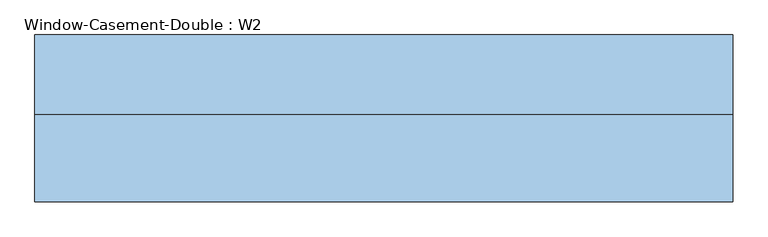
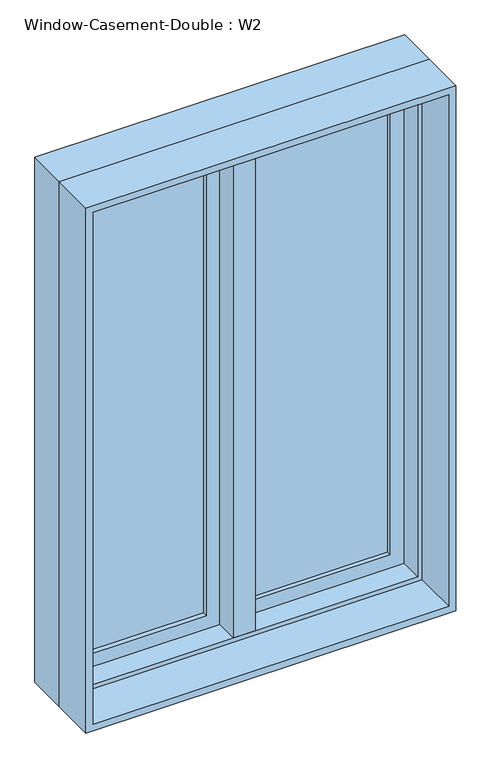
"""IFC4 building model written with IfcOpenShell, lengths in millimetres: window geometry, Window-Casement-Double : W2."""

import ifcopenshell
import ifcopenshell.guid

model = None  # the IFC model being written
_history = None  # IfcOwnerHistory: only IFC2X3 demands one
_inside = {}  # id of a spatial element -> (the spatial element, [elements in it])
_under = {}  # id of a project, library or spatial element -> (it, [spatial elements below it])
_declared = {}  # id of a project -> (the project, [libraries it declares])
_typed = {}  # id of a type object -> (the type object, [elements of that type])
_made_of = {}  # id of a material, layer set ... -> (it, [elements and type objects made of it])


def new_model(schema):
    """Start an empty IFC model of exactly this schema.

    Asked for "IFC4X3", IfcOpenShell would pick the latest addendum, in which some entities
    have other attributes; the version numbers below select the first issue.
    IFC2X3 requires an IfcOwnerHistory on every rooted entity: one is made here for all.
    """
    global model, _history
    if schema == "IFC4X3":
        model = ifcopenshell.file(schema_version=(4, 3, 0, 0))
    else:
        model = ifcopenshell.file(schema=schema)
    _inside.clear()
    _under.clear()
    _declared.clear()
    _typed.clear()
    _made_of.clear()
    _history = None
    if model.schema == "IFC2X3":
        org = make("IfcOrganization", Name="unknown")
        user = make(
            "IfcPersonAndOrganization",
            ThePerson=make("IfcPerson", FamilyName="unknown"),
            TheOrganization=org,
        )
        app = make(
            "IfcApplication",
            ApplicationDeveloper=org,
            Version="unknown",
            ApplicationFullName="unknown",
            ApplicationIdentifier="unknown",
        )
        _history = make(
            "IfcOwnerHistory",
            OwningUser=user,
            OwningApplication=app,
            ChangeAction="ADDED",
            CreationDate=0,
        )
    return model


def make(cls, **values):
    """One entity of the class cls with the attributes given. An attribute that is None is left unset."""
    return model.create_entity(
        cls, **{name: value for name, value in values.items() if value is not None}
    )


def rooted(cls, **values):
    """An entity with a GlobalId (a new one), such as an element, a storey or a relation."""
    return make(cls, GlobalId=ifcopenshell.guid.new(), OwnerHistory=_history, **values)


def si_unit(unit_type, name, prefix=None):
    """IfcSIUnit, for example si_unit("LENGTHUNIT", "METRE", prefix="MILLI")."""
    return make("IfcSIUnit", UnitType=unit_type, Prefix=prefix, Name=name)


def assignment(units):
    """IfcUnitAssignment: the units of a project."""
    return None if units is None else make("IfcUnitAssignment", Units=units)


def point(xyz):
    """IfcCartesianPoint."""
    return None if xyz is None else make("IfcCartesianPoint", Coordinates=xyz)


def direction(xyz):
    """IfcDirection."""
    return None if xyz is None else make("IfcDirection", DirectionRatios=xyz)


def frame(location, z_axis=None, x_axis=None):
    """IfcAxis2Placement3D, a coordinate frame: its origin and axes. An axis left out is left unset."""
    return make(
        "IfcAxis2Placement3D",
        Location=point(location),
        Axis=direction(z_axis),
        RefDirection=direction(x_axis),
    )


def origin():
    """The frame at (0, 0, 0) with its axes left unset."""
    return frame((0.0, 0.0, 0.0))


def place(relative_to, where):
    """IfcLocalPlacement: puts the frame where relative to a parent placement (None: the world)."""
    return make(
        "IfcLocalPlacement", PlacementRelTo=relative_to, RelativePlacement=where
    )


def context(
    kind, dimensions, precision=None, world=None, true_north=None, identifier=None
):
    """IfcGeometricRepresentationContext, for example the 3D "Model" context."""
    return make(
        "IfcGeometricRepresentationContext",
        ContextIdentifier=identifier,
        ContextType=kind,
        CoordinateSpaceDimension=dimensions,
        Precision=precision,
        WorldCoordinateSystem=world,
        TrueNorth=true_north,
    )


def project(units=None, contexts=None):
    """IfcProject with its units and contexts."""
    return rooted(
        "IfcProject",
        Name="project",
        RepresentationContexts=contexts,
        UnitsInContext=assignment(units),
    )


def spatial(cls, under=None, at=None, **own):
    """A site, building, storey or space (cls), placed at a placement, below another one or the project."""
    s = rooted(cls, ObjectPlacement=at, **own)
    if under is not None:
        _under.setdefault(under.id(), (under, []))[1].append(s)
    return s


def polyline(points):
    """IfcPolyline through the points."""
    return make("IfcPolyline", Points=[point(p) for p in points])


def outline(outer, holes=None, kind="AREA"):
    """IfcArbitraryClosedProfileDef: a profile drawn as a closed curve; with holes, ...WithVoids."""
    if holes is None:
        return make("IfcArbitraryClosedProfileDef", ProfileType=kind, OuterCurve=outer)
    return make(
        "IfcArbitraryProfileDefWithVoids",
        ProfileType=kind,
        OuterCurve=outer,
        InnerCurves=holes,
    )


def extrude(swept, where, along, depth):
    """IfcExtrudedAreaSolid: the profile swept, set in the frame where, extruded along a direction by depth."""
    return make(
        "IfcExtrudedAreaSolid",
        SweptArea=swept,
        Position=where,
        ExtrudedDirection=direction(along),
        Depth=depth,
    )


def faces_of(points, faces, orient=None, outer=None):
    """IfcFace entities. A face is a list of loops; a loop is a list of indices into points, from 0.

    orient and outer hold one flag for each loop. By default every Orientation is true, the
    first loop of a face is its IfcFaceOuterBound and the others are IfcFaceBound.
    """
    made = []
    for i, loops in enumerate(faces):
        bounds = []
        for j, loop in enumerate(loops):
            is_outer = j == 0 if outer is None else outer[i][j]
            bounds.append(
                make(
                    "IfcFaceOuterBound" if is_outer else "IfcFaceBound",
                    Bound=make("IfcPolyLoop", Polygon=[points[k] for k in loop]),
                    Orientation=True if orient is None else orient[i][j],
                )
            )
        made.append(make("IfcFace", Bounds=bounds))
    return made


def faceted_brep(points, faces, orient=None, outer=None, voids=None):
    """IfcFacetedBrep: a solid bounded by flat faces; with voids (closed shells), ...WithVoids."""
    shared = [point(p) for p in points]
    hull = make("IfcClosedShell", CfsFaces=faces_of(shared, faces, orient, outer))
    if voids is None:
        return make("IfcFacetedBrep", Outer=hull)
    return make(
        "IfcFacetedBrepWithVoids",
        Outer=hull,
        Voids=[
            make(cls, CfsFaces=faces_of(shared, fs, o, b)) for cls, fs, o, b in voids
        ],
    )


def shape(context_of_items, identifier, shape_type, items):
    """IfcShapeRepresentation: the items that make up one representation, for example the "Body"."""
    return make(
        "IfcShapeRepresentation",
        ContextOfItems=context_of_items,
        RepresentationIdentifier=identifier,
        RepresentationType=shape_type,
        Items=items,
    )


def source(mapping_origin, context_of_items, identifier, shape_type, items):
    """IfcRepresentationMap: a shape defined once, which mapped items show again and again."""
    return make(
        "IfcRepresentationMap",
        MappingOrigin=mapping_origin,
        MappedRepresentation=shape(context_of_items, identifier, shape_type, items),
    )


def transform(
    local_origin,
    x_axis=None,
    y_axis=None,
    z_axis=None,
    scale=None,
    scale2=None,
    scale3=None,
    uniform=True,
):
    """IfcCartesianTransformationOperator3D, or its non-uniform kind. x_axis, y_axis, z_axis: its Axis1, 2, 3."""
    if uniform:
        return make(
            "IfcCartesianTransformationOperator3D",
            Axis1=direction(x_axis),
            Axis2=direction(y_axis),
            LocalOrigin=point(local_origin),
            Scale=scale,
            Axis3=direction(z_axis),
        )
    return make(
        "IfcCartesianTransformationOperator3DnonUniform",
        Axis1=direction(x_axis),
        Axis2=direction(y_axis),
        LocalOrigin=point(local_origin),
        Scale=scale,
        Axis3=direction(z_axis),
        Scale2=scale2,
        Scale3=scale3,
    )


def mapped(mapping_source, mapping_target):
    """IfcMappedItem: shows the shape of a source again, moved by a transform."""
    return make(
        "IfcMappedItem", MappingSource=mapping_source, MappingTarget=mapping_target
    )


def made_of(thing, what):
    """Note that an element or type object is made of a material, layer set ...; save() writes the relation."""
    if what is not None:
        _made_of.setdefault(what.id(), (what, []))[1].append(thing)
    return thing


def element(
    cls,
    number,
    at=None,
    inside=None,
    cuts=None,
    type_object=None,
    material=None,
    context=None,
    identifier="Body",
    shape_type=None,
    held_by="IfcProductDefinitionShape",
    body=None,
    shapes=None,
    **own,
):
    """One element of the class cls, such as IfcWall. Its Tag is "e" and its number.

    at: its placement. inside: the storey or other place that contains it. cuts: it is an
    opening in that element (IfcRelVoidsElement). A single representation is given by context,
    identifier, shape_type and body (its items); several are given by shapes. held_by: the class
    of the entity that holds the representations. save() writes the other relations.
    """
    e = rooted(cls, Tag="e%d" % number, ObjectPlacement=at, **own)
    if body is not None:
        shapes = [shape(context, identifier, shape_type, body)]
    if shapes is not None:
        e.Representation = make(held_by, Representations=shapes)
    if inside is not None:
        _inside.setdefault(inside.id(), (inside, []))[1].append(e)
    if cuts is not None:
        rooted(
            "IfcRelVoidsElement", RelatingBuildingElement=cuts, RelatedOpeningElement=e
        )
    if type_object is not None:
        _typed.setdefault(type_object.id(), (type_object, []))[1].append(e)
    return made_of(e, material)


def aggregate(whole, parts):
    """IfcRelAggregates: a whole, such as a stair, and the parts it consists of."""
    return rooted("IfcRelAggregates", RelatingObject=whole, RelatedObjects=parts)


def save(model, path):
    """Write the relations noted so far, then the file.

    IfcRelAggregates (storeys below a building ...), IfcRelContainedInSpatialStructure (elements
    in a storey), IfcRelDefinesByType, IfcRelAssociatesMaterial and IfcRelDeclares: one each for
    every whole, place, type object, material and project.
    """
    for whole, parts in _under.values():
        aggregate(whole, parts)
    for where, things in _inside.values():
        rooted(
            "IfcRelContainedInSpatialStructure",
            RelatedElements=things,
            RelatingStructure=where,
        )
    for kind, things in _typed.values():
        rooted("IfcRelDefinesByType", RelatedObjects=things, RelatingType=kind)
    for what, things in _made_of.values():
        rooted("IfcRelAssociatesMaterial", RelatedObjects=things, RelatingMaterial=what)
    for by, libraries in _declared.values():
        rooted("IfcRelDeclares", RelatingContext=by, RelatedDefinitions=libraries)
    model.write(path)


def window_casement_double_w2_23809e8b(model_context):
    return source(origin(), model_context, "Body", "SolidModel", [
        faceted_brep([(9.525, 129.05, 2401.7), (-9.525, 129.05, 2401.7), (-9.525, 78.25, 2401.7), (9.525, 78.25, 2401.7), (9.525, 129.05, 927.1), (9.525, 78.25, 927.1), (-9.525, 78.25, 927.1), (-9.525, 129.05, 927.1), (-9.525, 78.25, 946.15), (-9.525, 78.25, 2382.65), (-30.1625, 78.25, 946.15), (-30.1625, 78.25, 2382.65), (-30.1625, 14.75, 946.15), (-30.1625, 14.75, 2382.65), (30.1625, 14.75, 946.15), (30.1625, 14.75, 2382.65), (30.1625, 78.25, 946.15), (30.1625, 78.25, 2382.65), (9.525, 78.25, 946.15), (9.525, 78.25, 2382.65)], [[[0, 1, 2, 3]], [[4, 5, 6, 7]], [[1, 0, 4, 7]], [[2, 1, 7, 6, 8, 9]], [[9, 8, 10, 11]], [[11, 10, 12, 13]], [[13, 12, 14, 15]], [[15, 14, 16, 17]], [[17, 16, 18, 19]], [[0, 3, 19, 18, 5, 4]], [[18, 8, 6, 5]], [[9, 19, 3, 2]], [[8, 18, 16, 14, 12, 10]], [[19, 9, 11, 13, 15, 17]]]),
        extrude(outline(polyline([(-66.675, 110.0), (-66.675, 103.65), (-430.15, 103.65), (-430.15, 110.0), (-66.675, 110.0)])), frame((0.0, 0.0, 984.25), z_axis=(0.0, 0.0, 1.0), x_axis=(1.0, 0.0, 0.0)), (0.0, 0.0, 1.0), 1360.3),
        extrude(outline(polyline([(-430.15, 90.95), (-430.15, 97.3), (-66.675, 97.3), (-66.675, 90.95), (-430.15, 90.95)])), frame((0.0, 0.0, 984.25), z_axis=(0.0, 0.0, 1.0), x_axis=(1.0, 0.0, 0.0)), (0.0, 0.0, 1.0), 1360.3),
        extrude(outline(polyline([(430.15, 110.0), (430.15, 103.65), (66.675, 103.65), (66.675, 110.0), (430.15, 110.0)])), frame((0.0, 0.0, 984.25), z_axis=(0.0, 0.0, 1.0), x_axis=(1.0, 0.0, 0.0)), (0.0, 0.0, 1.0), 1360.3),
        extrude(outline(polyline([(66.675, 90.95), (66.675, 97.3), (430.15, 97.3), (430.15, 90.95), (66.675, 90.95)])), frame((0.0, 0.0, 984.25), z_axis=(0.0, 0.0, 1.0), x_axis=(1.0, 0.0, 0.0)), (0.0, 0.0, 1.0), 1360.3),
        extrude(outline(polyline([(2401.7, -487.3), (927.1, -487.3), (927.1, -9.525), (2401.7, -9.525), (2401.7, -487.3)]), holes=[polyline([(2344.55, -66.675), (984.25, -66.675), (984.25, -430.15), (2344.55, -430.15), (2344.55, -66.675)])]), frame((0.0, 78.25, 0.0), z_axis=(0.0, 1.0, 0.0), x_axis=(0.0, 0.0, 1.0)), (0.0, 0.0, 1.0), 44.45),
        extrude(outline(polyline([(927.1, 487.3), (2401.7, 487.3), (2401.7, 9.525), (927.1, 9.525), (927.1, 487.3)]), holes=[polyline([(984.25, 66.675), (2344.55, 66.675), (2344.55, 430.15), (984.25, 430.15), (984.25, 66.675)])]), frame((0.0, 78.25, 0.0), z_axis=(0.0, 1.0, 0.0), x_axis=(0.0, 0.0, 1.0)), (0.0, 0.0, 1.0), 44.45),
        extrude(outline(polyline([(2414.4, -500.0), (914.4, -500.0), (914.4, 500.0), (2414.4, 500.0), (2414.4, -500.0)]), holes=[polyline([(2395.35, 480.95), (933.45, 480.95), (933.45, -480.95), (2395.35, -480.95), (2395.35, 480.95)])]), frame((0.0, -110.0, 0.0), z_axis=(0.0, 1.0, 0.0), x_axis=(0.0, 0.0, 1.0)), (0.0, 0.0, 1.0), 124.75),
        faceted_brep([(468.25, 78.25, 2382.65), (468.25, 14.75, 2382.65), (-468.25, 14.75, 2382.65), (-468.25, 78.25, 2382.65), (487.3, 129.05, 2401.7), (487.3, 78.25, 2401.7), (-487.3, 78.25, 2401.7), (-487.3, 129.05, 2401.7), (500.0, 14.75, 2414.4), (500.0, 129.05, 2414.4), (-500.0, 129.05, 2414.4), (-500.0, 14.75, 2414.4), (-468.25, 14.75, 946.15), (-468.25, 78.25, 946.15), (-487.3, 78.25, 927.1), (-487.3, 129.05, 927.1), (-500.0, 129.05, 914.4), (-500.0, 14.75, 914.4), (468.25, 14.75, 946.15), (468.25, 78.25, 946.15), (487.3, 78.25, 927.1), (487.3, 129.05, 927.1), (500.0, 129.05, 914.4), (500.0, 14.75, 914.4)], [[[0, 1, 2, 3]], [[4, 5, 6, 7]], [[8, 9, 10, 11]], [[3, 2, 12, 13]], [[7, 6, 14, 15]], [[11, 10, 16, 17]], [[13, 12, 18, 19]], [[15, 14, 20, 21]], [[17, 16, 22, 23]], [[11, 17, 23, 8], [1, 18, 12, 2]], [[19, 18, 1, 0]], [[5, 20, 14, 6], [3, 13, 19, 0]], [[21, 20, 5, 4]], [[23, 22, 9, 8]], [[9, 22, 16, 10], [7, 15, 21, 4]]]),
    ])


if __name__ == "__main__":
    model = new_model("IFC4")
    model_context = context("Model", 3, world=origin())
    ifc_project = project(units=[si_unit("LENGTHUNIT", "METRE", prefix="MILLI")], contexts=[model_context])
    site = spatial("IfcSite", under=ifc_project)
    building = spatial("IfcBuilding", under=site)
    placement = place(None, origin())
    window_casement_double_w2_shape = window_casement_double_w2_23809e8b(model_context)
    element("IfcWindow", 1, ObjectType="Window-Casement-Double : W2", at=placement, inside=building, context=model_context, shape_type="MappedRepresentation", body=[
        mapped(window_casement_double_w2_shape, transform((0.0, 0.0, 0.0), x_axis=(1.0, 0.0, 0.0), y_axis=(0.0, 1.0, 0.0), z_axis=(0.0, 0.0, 1.0))),
    ])
    save(model, "model.ifc")

# Revit data of these elements
# Type "Window-Casement-Double : W2"
#   Type Mark = "28"
#   Fire Rating = "0.5h"
#   Assembly Code = "B2020100"
#   Analytic Construction = "Double glazing - domestic"
#   Frame Extension [instance default] = 0.635 cm
#   Window Inset [instance default] = 0 cm
#   Wall Thickness [instance default] = 15.24 cm
#   Interior Wall Closure [instance default] = 5.715 cm
#   Half Width = 50 cm
#   Visual Light Transmittance = 0.81
#   Thermal Resistance (R) = 0.319569 (m²·K)/W
#   Solar Heat Gain Coefficient = 0.76
#   Rough Width = 101.27 cm
#   Rough Height = 151.27 cm
#   Height = 150 cm
#   Heat Transfer Coefficient (U) = 3.12929 W/(m²·K)
#   Exterior Wall Closure [instance default] = 3.175 cm
#   Extension Jamb [instance default] = 5.715 cm
#   Default Sill Height = 91.44 cm
#   Width = 100 cm
#   Muntin Visibility = yes
#   Interior Trim Visibility [instance default] = yes
#   Exterior Trim Visibility [instance default] = yes
#   Extension Jamb Visibility [instance default] = yes
#   Interior Trim Material = Wood - Stained
#   Muntin Pattern = Muntin Pattern_2x2 : Muntin Pattern_2x2
#   Interior Trim = Trim-Window-Interior-Flat : Picture Frame
#   Interior Frame Material = Wood - Stained
#   Glass Panel Material = Glass
#   Exterior Trim Material = Clad - White
#   Exterior Trim = Trim-Window-Exterior-Flat : with Sill
#   Exterior Frame Material = Clad - White
#   Wall Closure = (empty or 0)
# Element 1 (IfcWindow, "Window-Casement-Double : W2")
#   Wall Thickness = 22 cm
#   Extension Jamb = 12.475 cm
#   Materials on its faces: "Wood - Stained", "Glass", "Clad - White"
# Materials
#   "Wood - Stained": class "Wood", colour RGB 224 178 126, transparency 0, Cost = 0
#   "Glass": class "Glass", colour RGB 0 128 192, transparency 0.9, Description = "Soda Lime Glass", Cost = 0
#   "Clad - White": class "Wood", colour RGB 242 242 238, transparency 0, Cost = 0
